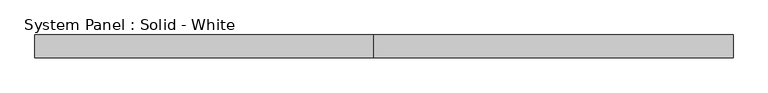
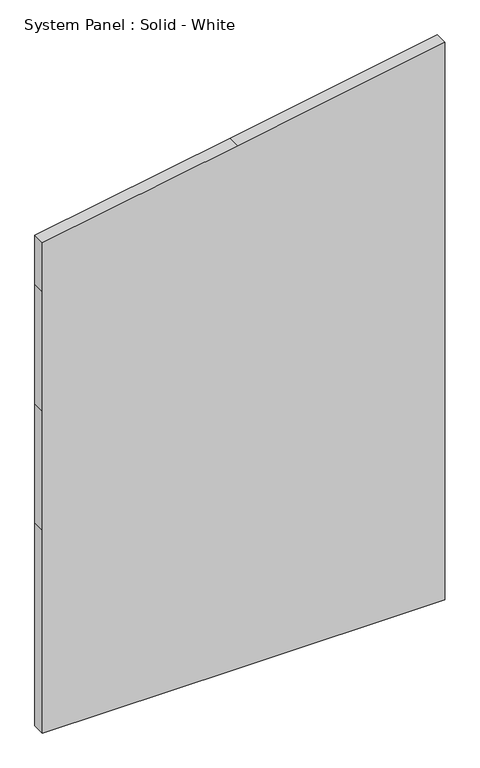
"""IFC4 building model written with IfcOpenShell, lengths in millimetres: plate geometry, System Panel : Solid - White."""

from ifc_helpers import new_model, si_unit, frame, origin, place, context, project, spatial, polyline, outline, extrude, source, transform, mapped, element, save


def system_panel_solid_white_d0de5aa5(model_context):
    return source(origin(), model_context, "Body", "SweptSolid", [
        extrude(outline(polyline([(0.0, -974.1121469), (0.0, -39.6038136), (0.0, 974.1121469), (1038.2580051, 974.1121469), (1647.8580051, 974.1121469), (2257.4580051, 974.1121469), (2852.499686, 974.1121469), (2675.6985089, -28.5771543), (2508.9751785, -974.1121469), (2257.4580051, -974.1121469), (1647.8580051, -974.1121469), (1038.2580051, -974.1121469), (0.0, -974.1121469)])), frame((0.0, -44.45, 0.0), z_axis=(0.0, 1.0, 0.0), x_axis=(0.0, 0.0, 1.0)), (0.0, 0.0, 1.0), 63.5),
    ])


if __name__ == "__main__":
    model = new_model("IFC4")
    model_context = context("Model", 3, world=origin())
    ifc_project = project(units=[si_unit("LENGTHUNIT", "METRE", prefix="MILLI")], contexts=[model_context])
    site = spatial("IfcSite", under=ifc_project)
    building = spatial("IfcBuilding", under=site)
    placement = place(None, origin())
    system_panel_solid_white_shape = system_panel_solid_white_d0de5aa5(model_context)
    element("IfcPlate", 1, ObjectType="System Panel : Solid - White", at=placement, inside=building, context=model_context, shape_type="MappedRepresentation", body=[
        mapped(system_panel_solid_white_shape, transform((0.0, 0.0, 0.0), x_axis=(1.0, 0.0, 0.0), y_axis=(0.0, 1.0, 0.0), z_axis=(0.0, 0.0, 1.0))),
    ])
    save(model, "model.ifc")

# Revit data of these elements
# Element 1 (IfcPlate, "System Panel : Solid - White")
#   Materials on its faces: "White Panel"
# Materials
#   "White Panel": class "Unassigned", colour RGB 255 255 255, transparency 0
